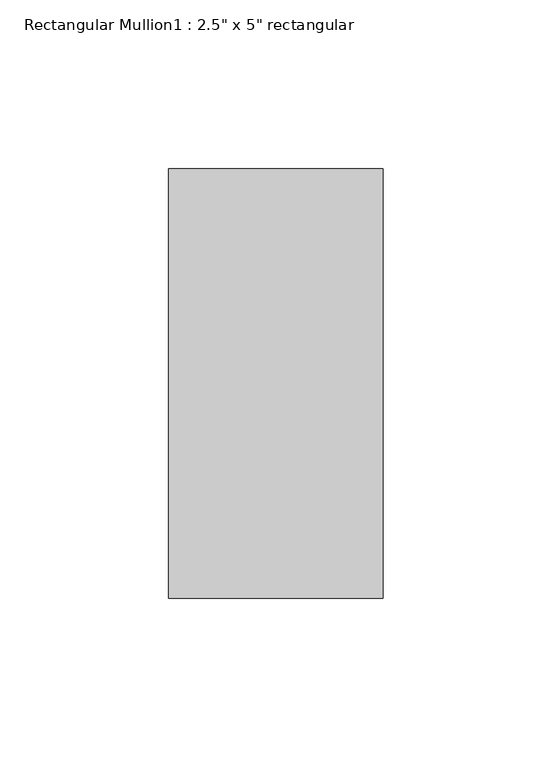
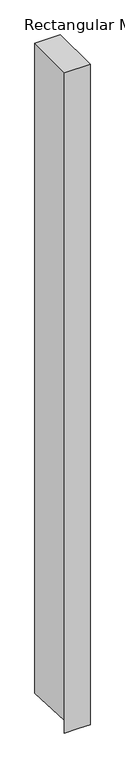
"""IFC4 building model written with IfcOpenShell, lengths in millimetres: member geometry."""

from ifc_helpers import new_model, si_unit, origin, place, context, project, spatial, faceted_brep, source, transform, mapped, element, save


def member_fbbd287a(model_context):
    return source(origin(), model_context, "Body", "Brep", [
        faceted_brep([(31.75, 63.5, 0.0), (-31.75, 63.5, 0.0), (-31.75, -63.5, 0.0), (31.75, -63.5, 0.0), (31.75, 63.5, -1705.0231573), (0.0, 63.5, -1705.0231573), (-31.75, 63.5, -1705.0231573), (-31.75, -62.1974623, -1700.0584389), (-31.75, -63.5, -1733.0362781), (0.0, -63.5, -1733.0362781), (31.75, -63.5, -1733.0362781), (31.75, -62.1974623, -1700.0584389), (0.0, -62.1974623, -1700.0584389)], [[[0, 1, 2, 3]], [[1, 0, 4, 5, 6]], [[2, 1, 6, 7, 8]], [[3, 2, 8, 9, 10]], [[0, 3, 10, 11, 4]], [[4, 11, 12, 5]], [[11, 10, 9, 12]], [[9, 8, 7, 12]], [[7, 6, 5, 12]]]),
    ])


if __name__ == "__main__":
    model = new_model("IFC4")
    model_context = context("Model", 3, world=origin())
    ifc_project = project(units=[si_unit("LENGTHUNIT", "METRE", prefix="MILLI")], contexts=[model_context])
    site = spatial("IfcSite", under=ifc_project)
    building = spatial("IfcBuilding", under=site)
    placement = place(None, origin())
    member_shape = member_fbbd287a(model_context)
    element("IfcMember", 1, ObjectType="Rectangular Mullion1 : 2.5\" x 5\" rectangular", at=placement, inside=building, context=model_context, shape_type="MappedRepresentation", body=[
        mapped(member_shape, transform((0.0, 0.0, 0.0), x_axis=(1.0, 0.0, 0.0), y_axis=(0.0, 1.0, 0.0), z_axis=(0.0, 0.0, 1.0))),
    ])
    save(model, "model.ifc")

# Revit data of these elements
# Type "Rectangular Mullion1 : 2.5\" x 5\" rectangular"
#   built-in parameter 1007304 = 0.416667 (stored number, unit not read)
#   built-in parameter 1007301 = 0.104167 (stored number, unit not read)
#   built-in parameter 1007300 = 0.104167 (stored number, unit not read)
# Element 1 (IfcMember, "Rectangular Mullion1 : 2.5\" x 5\" rectangular")
#   Materials on its faces: "support-frame"
# Materials
#   "support-frame": class "Unassigned", colour RGB 233 233 233, transparency 0, Cost = 0
